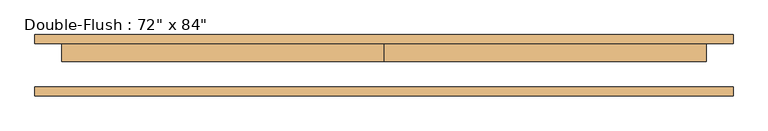
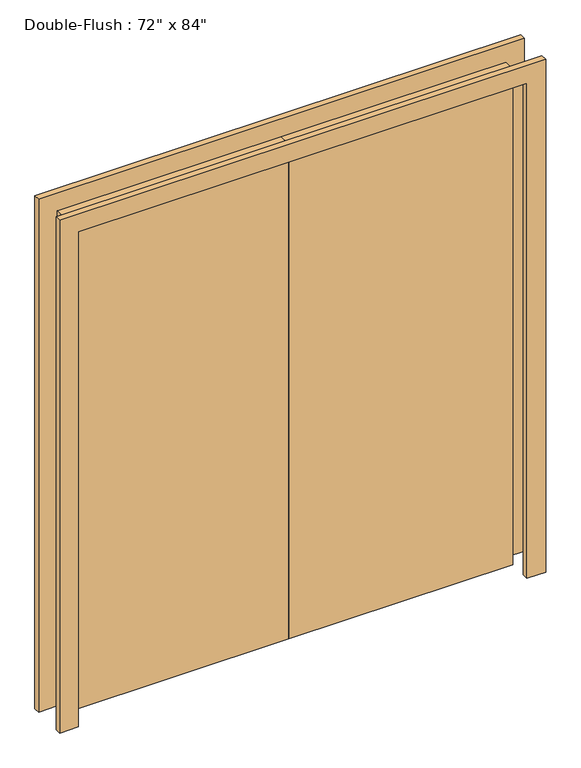
"""IFC4 building model written with IfcOpenShell, lengths in millimetres: door geometry."""

from ifc_helpers import new_model, si_unit, frame, origin, origin_with_axes, place, context, project, spatial, polyline, outline, extrude, source, transform, mapped, element, save


def door_1edc655c(model_context):
    return source(origin(), model_context, "Body", "SweptSolid", [
        extrude(outline(polyline([(0.0, 61.9125), (914.4, 61.9125), (914.4, 11.1125), (0.0, 11.1125), (0.0, 61.9125)])), origin_with_axes(), (0.0, 0.0, 1.0), 2133.6),
        extrude(outline(polyline([(-914.4, 61.9125), (0.0, 61.9125), (0.0, 11.1125), (-914.4, 11.1125), (-914.4, 61.9125)])), origin_with_axes(), (0.0, 0.0, 1.0), 2133.6),
        extrude(outline(polyline([(2133.6, -914.4), (2133.6, 914.4), (0.0, 914.4), (0.0, 990.6), (2209.8, 990.6), (2209.8, -990.6), (0.0, -990.6), (0.0, -914.4), (2133.6, -914.4)])), frame((0.0, -87.3125, 0.0), z_axis=(0.0, 1.0, 0.0), x_axis=(0.0, 0.0, 1.0)), (0.0, 0.0, 1.0), 25.4),
        extrude(outline(polyline([(2133.6, -914.4), (2133.6, 914.4), (0.0, 914.4), (0.0, 990.6), (2209.8, 990.6), (2209.8, -990.6), (0.0, -990.6), (0.0, -914.4), (2133.6, -914.4)])), frame((0.0, 61.9125, 0.0), z_axis=(0.0, 1.0, 0.0), x_axis=(0.0, 0.0, 1.0)), (0.0, 0.0, 1.0), 25.4),
    ])


if __name__ == "__main__":
    model = new_model("IFC4")
    model_context = context("Model", 3, world=origin())
    ifc_project = project(units=[si_unit("LENGTHUNIT", "METRE", prefix="MILLI")], contexts=[model_context])
    site = spatial("IfcSite", under=ifc_project)
    building = spatial("IfcBuilding", under=site)
    placement = place(None, origin())
    door_shape = door_1edc655c(model_context)
    element("IfcDoor", 1, ObjectType="Double-Flush : 72\" x 84\"", at=placement, inside=building, context=model_context, shape_type="MappedRepresentation", body=[
        mapped(door_shape, transform((0.0, 0.0, 0.0), x_axis=(1.0, 0.0, 0.0), y_axis=(0.0, 1.0, 0.0), z_axis=(0.0, 0.0, 1.0))),
    ])
    save(model, "model.ifc")

# Revit data of these elements
# Type "Double-Flush : 72\" x 84\""
#   Type Mark = "14"
#   Construction Type = "I"
#   Assembly Code = "C1020"
#   Thickness = 0' - 2"
#   Height = 7' - 0"
#   Trim Projection Ext = 0' - 1"
#   Trim Projection Int = 0' - 1"
#   Trim Width = 0' - 3"
#   Width = 6' - 0"
#   Door Material = Door - Panel
#   Frame Material = Door - Frame
#   Function = (empty or 0)
#   Wall Closure = (empty or 0)
# Element 1 (IfcDoor, "Double-Flush : 72\" x 84\"")
#   Materials on its faces: "Door - Frame", "Door - Panel"
# Materials
#   "Door - Panel": class "Wood", colour RGB 210 159 95, transparency 0
#   "Door - Frame": class "Miscellaneous", colour RGB 118 70 51, transparency 0
